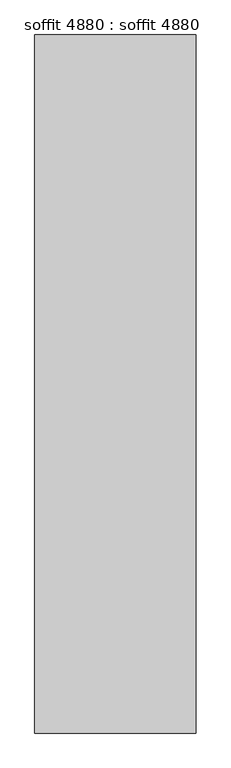
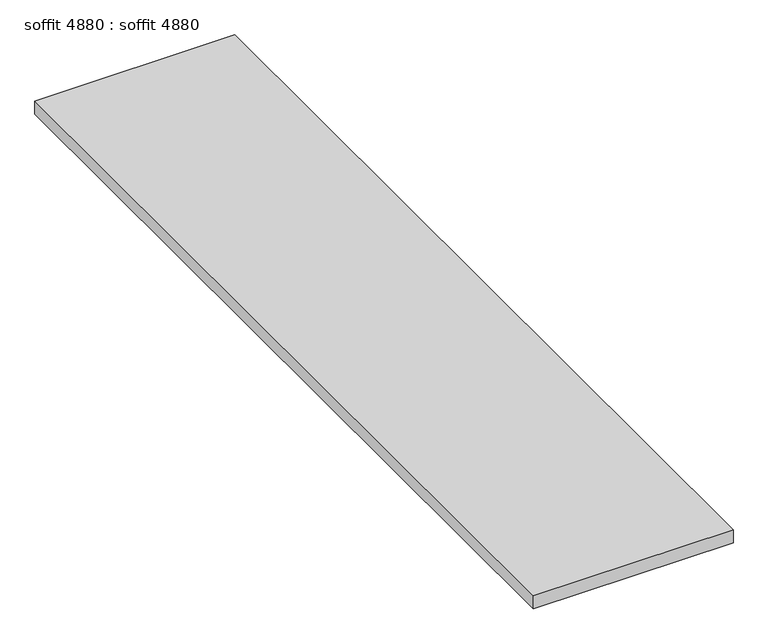
"""IFC4 building model written with IfcOpenShell, lengths in millimetres: proxy geometry, soffit 4880 : soffit 4880."""

from ifc_helpers import new_model, si_unit, frame, origin, place, context, project, spatial, polyline, outline, extrude, source, transform, mapped, element, save


def soffit_4880_soffit_4880_d099dfd0(model_context):
    return source(origin(), model_context, "Body", "SweptSolid", [
        extrude(outline(polyline([(-468.8598633, -1052.8906574), (-931.3315411, -1052.8906574), (-931.3315411, 947.1093426), (-468.8598633, 947.1093426), (-468.8598633, -1052.8906574)])), frame((0.0, 0.0, 42101.9016246), z_axis=(0.0, 0.0, 1.0), x_axis=(1.0, 0.0, 0.0)), (0.0, 0.0, 1.0), 31.9020447),
    ])


if __name__ == "__main__":
    model = new_model("IFC4")
    model_context = context("Model", 3, world=origin())
    ifc_project = project(units=[si_unit("LENGTHUNIT", "METRE", prefix="MILLI")], contexts=[model_context])
    site = spatial("IfcSite", under=ifc_project)
    building = spatial("IfcBuilding", under=site)
    placement = place(None, origin())
    soffit_4880_soffit_4880_shape = soffit_4880_soffit_4880_d099dfd0(model_context)
    element("IfcBuildingElementProxy", 1, Name="soffit 4880 : soffit 4880", ObjectType="soffit 4880 : soffit 4880", at=placement, inside=building, context=model_context, shape_type="MappedRepresentation", body=[
        mapped(soffit_4880_soffit_4880_shape, transform((0.0, 0.0, 0.0), x_axis=(1.0, 0.0, 0.0), y_axis=(0.0, 1.0, 0.0), z_axis=(0.0, 0.0, 1.0))),
    ])
    save(model, "model.ifc")

# Revit data of these elements
# Type "soffit 4880 : soffit 4880"
#   NameOverride = "soffit"
# Element 1 (IfcBuildingElementProxy, "soffit 4880 : soffit 4880")
#   Materials on its faces: "WHITE OAK (SPEC T.B.D.) OVER BUILDING WRAP"
# Materials
#   "WHITE OAK (SPEC T.B.D.) OVER BUILDING WRAP": class "Unassigned", colour RGB 227 188 136, transparency 0, Cost = 0
